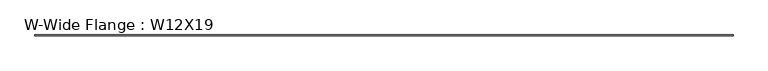
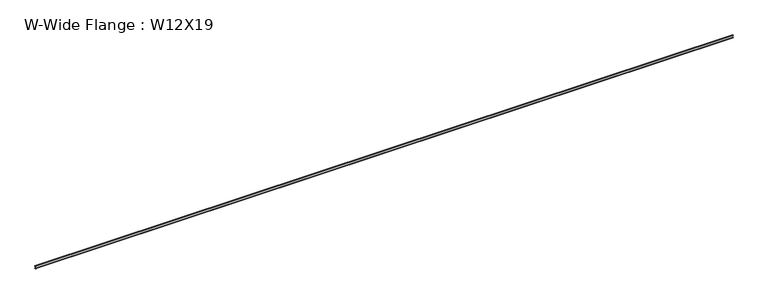
"""IFC4 building model written with IfcOpenShell, lengths in millimetres: beam geometry, W-Wide Flange : W12X19."""

from ifc_helpers import new_model, si_unit, point, frame, frame_2d, origin, place, context, project, spatial, polyline, circle_curve, trimmed, segment, composite_curve, outline, extrude, source, transform, mapped, element, save


def w_wide_flange_w12x19_f5d0d782(model_context):
    return source(origin(), model_context, "Body", "SweptSolid", [
        extrude(outline(composite_curve([segment(polyline([(50.927, -146.05), (50.927, -154.94), (-50.927, -154.94), (-50.927, -146.05), (-16.3195, -146.05)]), True, "CONTINUOUS"), segment(trimmed(circle_curve(frame_2d((-16.3195, -132.715)), 13.335), [point((-16.3195, -146.05))], [point((-2.9845, -132.715))], True, "CARTESIAN"), True, "CONTINUOUS"), segment(polyline([(-2.9845, -132.715), (-2.9845, 132.715)]), True, "CONTINUOUS"), segment(trimmed(circle_curve(frame_2d((-16.3195, 132.715)), 13.335), [point((-2.9845, 132.715))], [point((-16.3195, 146.05))], True, "CARTESIAN"), True, "CONTINUOUS"), segment(polyline([(-16.3195, 146.05), (-50.927, 146.05), (-50.927, 154.94), (50.927, 154.94), (50.927, 146.05), (16.3195, 146.05)]), True, "CONTINUOUS"), segment(trimmed(circle_curve(frame_2d((16.3195, 132.715)), 13.335), [point((16.3195, 146.05))], [point((2.9845, 132.715))], True, "CARTESIAN"), True, "CONTINUOUS"), segment(polyline([(2.9845, 132.715), (2.9845, -132.715)]), True, "CONTINUOUS"), segment(trimmed(circle_curve(frame_2d((16.3195, -132.715)), 13.335), [point((2.9845, -132.715))], [point((16.3195, -146.05))], True, "CARTESIAN"), True, "CONTINUOUS"), segment(polyline([(16.3195, -146.05), (50.927, -146.05)]), True, "CONTINUOUS")], self_intersect=False)), frame((-44073.7625, 0.0, 0.0), z_axis=(1.0, 0.0, 0.0), x_axis=(0.0, 1.0, 0.0)), (0.0, 0.0, 1.0), 88074.5),
    ])


if __name__ == "__main__":
    model = new_model("IFC4")
    model_context = context("Model", 3, world=origin())
    ifc_project = project(units=[si_unit("LENGTHUNIT", "METRE", prefix="MILLI")], contexts=[model_context])
    site = spatial("IfcSite", under=ifc_project)
    building = spatial("IfcBuilding", under=site)
    placement = place(None, origin())
    w_wide_flange_w12x19_shape = w_wide_flange_w12x19_f5d0d782(model_context)
    element("IfcBeam", 1, ObjectType="W-Wide Flange : W12X19", at=placement, inside=building, context=model_context, shape_type="MappedRepresentation", body=[
        mapped(w_wide_flange_w12x19_shape, transform((0.0, 0.0, 0.0), x_axis=(1.0, 0.0, 0.0), y_axis=(0.0, 1.0, 0.0), z_axis=(0.0, 0.0, 1.0))),
    ])
    save(model, "model.ifc")

# Revit data of these elements
# Type "W-Wide Flange : W12X19"
#   Assembly Code = "B10"
#   W = 19
#   Length [instance default] = 5' - 0"
#   bf = 0' - 4.01"
#   d = 1' - 0.2"
#   k = 0' - 0 7/8"
#   k2 = 0' - 0.525"
#   tf = 0' - 0.35"
#   tw = 0' - 0.235"
#   A = 0.0386806 SF
#   Structural Material [instance default] = Steel ASTM A992
# Element 1 (IfcBeam, "W-Wide Flange : W12X19")
#   Structural Material = STRUCTURAL STEEL - SEE STRUCT. DWGS
#   Materials on its faces: "STRUCTURAL STEEL - SEE STRUCT. DWGS"
# Materials
#   "Steel ASTM A992": class "Metal", colour RGB 199 199 199, transparency 0, Description = "Structural steel 50ksi", Cost = 0
#   "STRUCTURAL STEEL - SEE STRUCT. DWGS": class "Metal", colour RGB 137 146 153, transparency 0, Description = "Steel, mill finish", Cost = 0
